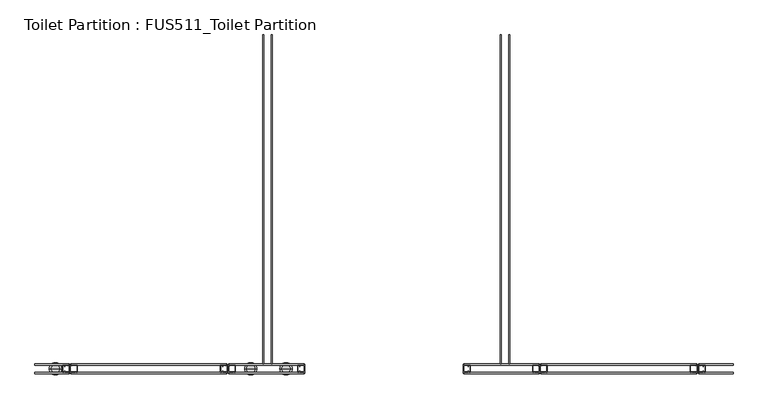
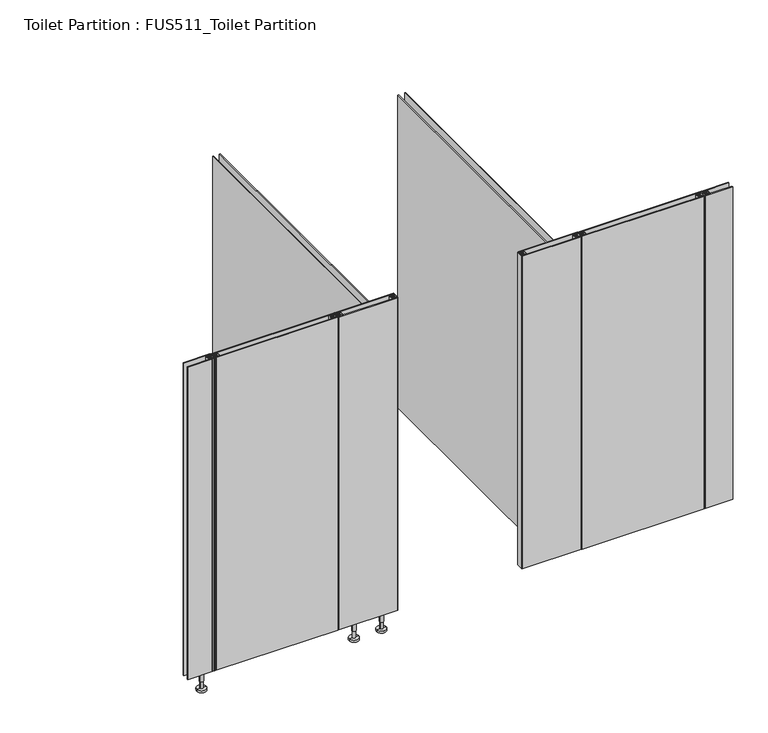
"""IFC4 building model written with IfcOpenShell, lengths in millimetres: furniture geometry, Toilet Partition : FUS511_Toilet Partition."""

from ifc_helpers import new_model, si_unit, point, frame, frame_2d, origin, place, context, project, spatial, polyline, circle_curve, trimmed, segment, composite_curve, outline, extrude, source, transform, mapped, element, save
from ifc_brep_helpers import plane_surface, cylinder_surface, advanced_brep


def toilet_partition_fus511_toilet_partition_2ff23377(model_context):
    return source(origin(), model_context, "Body", "SolidModel", [
        advanced_brep(
        [(-443.912605, 474.714347, 104.1461397), (-412.6687631, 474.714347, 104.1461397), (-412.6687631, 474.714347, 101.0217555), (-443.912605, 474.714347, 101.0217555), (-454.3272189, 474.714347, 0.0), (-402.2541491, 474.714347, 0.0), (-428.290684, 474.714347, 0.0), (-454.3272189, 474.714347, 10.414614), (-402.2541491, 474.714347, 10.414614), (-436.1016445, 474.714347, 10.414614), (-420.4797235, 474.714347, 10.414614), (-436.1016445, 474.714347, 52.0730698), (-420.4797235, 474.714347, 52.0730698), (-438.705298, 474.714347, 52.0730698), (-417.8760701, 474.714347, 52.0730698), (-438.705298, 474.714347, 101.0217555), (-417.8760701, 474.714347, 101.0217555), (-445.9955278, 474.714347, 104.1461397), (-410.5858403, 474.714347, 104.1461397), (-445.9955278, 474.714347, 110.394908), (-410.5858403, 474.714347, 110.394908), (-428.290684, 474.714347, 110.394908)],
        [
            (0, 1, circle_curve(frame((-428.290684, 474.714347, 104.1461397), z_axis=(0.0, 0.0, -1.0), x_axis=(1.0, 0.0, 0.0)), 15.6219209)),
            (1, 2),
            (2, 3, circle_curve(frame((-428.290684, 474.714347, 101.0217555), z_axis=(0.0, 0.0, 1.0), x_axis=(1.0, 0.0, 0.0)), 15.6219209)),
            (3, 0),
            (1, 0, circle_curve(frame((-428.290684, 474.714347, 104.1461397), z_axis=(0.0, 0.0, -1.0), x_axis=(1.0, 0.0, 0.0)), 15.6219209)),
            (3, 2, circle_curve(frame((-428.290684, 474.714347, 101.0217555), z_axis=(0.0, 0.0, 1.0), x_axis=(1.0, 0.0, 0.0)), 15.6219209)),
            (4, 5, circle_curve(frame((-428.290684, 474.714347, 0.0), z_axis=(0.0, 0.0, -1.0), x_axis=(1.0, 0.0, 0.0)), 26.0365349)),
            (5, 6),
            (6, 4),
            (5, 4, circle_curve(frame((-428.290684, 474.714347, 0.0), z_axis=(0.0, 0.0, -1.0), x_axis=(1.0, 0.0, 0.0)), 26.0365349)),
            (7, 8, circle_curve(frame((-428.290684, 474.714347, 10.414614), z_axis=(0.0, 0.0, -1.0), x_axis=(1.0, 0.0, 0.0)), 26.0365349)),
            (8, 5),
            (4, 7),
            (8, 7, circle_curve(frame((-428.290684, 474.714347, 10.414614), z_axis=(0.0, 0.0, -1.0), x_axis=(1.0, 0.0, 0.0)), 26.0365349)),
            (9, 10, circle_curve(frame((-428.290684, 474.714347, 10.414614), z_axis=(0.0, 0.0, -1.0), x_axis=(1.0, 0.0, 0.0)), 7.8109605)),
            (10, 8),
            (7, 9),
            (10, 9, circle_curve(frame((-428.290684, 474.714347, 10.414614), z_axis=(0.0, 0.0, -1.0), x_axis=(1.0, 0.0, 0.0)), 7.8109605)),
            (11, 12, circle_curve(frame((-428.290684, 474.714347, 52.0730698), z_axis=(0.0, 0.0, -1.0), x_axis=(1.0, 0.0, 0.0)), 7.8109605)),
            (12, 10),
            (9, 11),
            (12, 11, circle_curve(frame((-428.290684, 474.714347, 52.0730698), z_axis=(0.0, 0.0, -1.0), x_axis=(1.0, 0.0, 0.0)), 7.8109605)),
            (13, 14, circle_curve(frame((-428.290684, 474.714347, 52.0730698), z_axis=(0.0, 0.0, -1.0), x_axis=(1.0, 0.0, 0.0)), 10.414614)),
            (14, 12),
            (11, 13),
            (14, 13, circle_curve(frame((-428.290684, 474.714347, 52.0730698), z_axis=(0.0, 0.0, -1.0), x_axis=(1.0, 0.0, 0.0)), 10.414614)),
            (15, 16, circle_curve(frame((-428.290684, 474.714347, 101.0217555), z_axis=(0.0, 0.0, -1.0), x_axis=(1.0, 0.0, 0.0)), 10.414614)),
            (16, 14),
            (13, 15),
            (16, 15, circle_curve(frame((-428.290684, 474.714347, 101.0217555), z_axis=(0.0, 0.0, -1.0), x_axis=(1.0, 0.0, 0.0)), 10.414614)),
            (2, 16),
            (15, 3),
            (17, 18, circle_curve(frame((-428.290684, 474.714347, 104.1461397), z_axis=(0.0, 0.0, -1.0), x_axis=(1.0, 0.0, 0.0)), 17.7048437)),
            (18, 1),
            (0, 17),
            (18, 17, circle_curve(frame((-428.290684, 474.714347, 104.1461397), z_axis=(0.0, 0.0, -1.0), x_axis=(1.0, 0.0, 0.0)), 17.7048437)),
            (19, 20, circle_curve(frame((-428.290684, 474.714347, 110.394908), z_axis=(0.0, 0.0, -1.0), x_axis=(1.0, 0.0, 0.0)), 17.7048437)),
            (20, 18),
            (17, 19),
            (20, 19, circle_curve(frame((-428.290684, 474.714347, 110.394908), z_axis=(0.0, 0.0, -1.0), x_axis=(1.0, 0.0, 0.0)), 17.7048437)),
            (21, 20),
            (19, 21),
        ],
        [
            cylinder_surface(frame((-428.290684, 474.714347, 190.0), z_axis=(0.0, 0.0, 1.0), x_axis=(1.0, 0.0, 0.0)), 15.6219209),
            plane_surface(frame((-428.290684, 474.714347, 0.0), z_axis=(0.0, 0.0, -1.0), x_axis=(1.0, 0.0, 0.0))),
            cylinder_surface(frame((-428.290684, 474.714347, 190.0), z_axis=(0.0, 0.0, 1.0), x_axis=(1.0, 0.0, 0.0)), 26.0365349),
            plane_surface(frame((-428.290684, 474.714347, 10.414614), z_axis=(0.0, 0.0, 1.0), x_axis=(1.0, 0.0, 0.0))),
            cylinder_surface(frame((-428.290684, 474.714347, 190.0), z_axis=(0.0, 0.0, 1.0), x_axis=(1.0, 0.0, 0.0)), 7.8109605),
            plane_surface(frame((-428.290684, 474.714347, 52.0730698), z_axis=(0.0, 0.0, -1.0), x_axis=(1.0, 0.0, 0.0))),
            cylinder_surface(frame((-428.290684, 474.714347, 190.0), z_axis=(0.0, 0.0, 1.0), x_axis=(1.0, 0.0, 0.0)), 10.414614),
            plane_surface(frame((-428.290684, 474.714347, 101.0217555), z_axis=(0.0, 0.0, -1.0), x_axis=(1.0, 0.0, 0.0))),
            plane_surface(frame((-428.290684, 474.714347, 104.1461397), z_axis=(0.0, 0.0, -1.0), x_axis=(1.0, 0.0, 0.0))),
            cylinder_surface(frame((-428.290684, 474.714347, 190.0), z_axis=(0.0, 0.0, 1.0), x_axis=(1.0, 0.0, 0.0)), 17.7048437),
            plane_surface(frame((-428.290684, 474.714347, 110.394908), z_axis=(0.0, 0.0, 1.0), x_axis=(1.0, 0.0, 0.0))),
        ],
        [
            (0, [[1, 2, 3, 4]]),
            (0, [[5, -4, 6, -2]]),
            (1, [[7, 8, 9]]),
            (1, [[10, -9, -8]]),
            (2, [[11, 12, -7, 13]]),
            (2, [[14, -13, -10, -12]]),
            (3, [[15, 16, -11, 17]]),
            (3, [[18, -17, -14, -16]]),
            (4, [[19, 20, -15, 21]]),
            (4, [[22, -21, -18, -20]]),
            (5, [[23, 24, -19, 25]]),
            (5, [[26, -25, -22, -24]]),
            (6, [[27, 28, -23, 29]]),
            (6, [[30, -29, -26, -28]]),
            (7, [[-3, 31, -27, 32]]),
            (7, [[-6, -32, -30, -31]]),
            (8, [[33, 34, -1, 35]]),
            (8, [[36, -35, -5, -34]]),
            (9, [[37, 38, -33, 39]]),
            (9, [[40, -39, -36, -38]]),
            (10, [[41, -37, 42]]),
            (10, [[-42, -40, -41]]),
        ],
    ),
        advanced_brep(
        [(-593.912605, 474.714347, 104.1461397), (-562.6687631, 474.714347, 104.1461397), (-562.6687631, 474.714347, 101.0217555), (-593.912605, 474.714347, 101.0217555), (-604.3272189, 474.714347, 0.0), (-552.2541491, 474.714347, 0.0), (-578.290684, 474.714347, 0.0), (-604.3272189, 474.714347, 10.414614), (-552.2541491, 474.714347, 10.414614), (-586.1016445, 474.714347, 10.414614), (-570.4797235, 474.714347, 10.414614), (-586.1016445, 474.714347, 52.0730698), (-570.4797235, 474.714347, 52.0730698), (-588.705298, 474.714347, 52.0730698), (-567.8760701, 474.714347, 52.0730698), (-588.705298, 474.714347, 101.0217555), (-567.8760701, 474.714347, 101.0217555), (-595.9955278, 474.714347, 104.1461397), (-560.5858403, 474.714347, 104.1461397), (-595.9955278, 474.714347, 110.394908), (-560.5858403, 474.714347, 110.394908), (-578.290684, 474.714347, 110.394908)],
        [
            (0, 1, circle_curve(frame((-578.290684, 474.714347, 104.1461397), z_axis=(0.0, 0.0, -1.0), x_axis=(1.0, 0.0, 0.0)), 15.6219209)),
            (1, 2),
            (2, 3, circle_curve(frame((-578.290684, 474.714347, 101.0217555), z_axis=(0.0, 0.0, 1.0), x_axis=(1.0, 0.0, 0.0)), 15.6219209)),
            (3, 0),
            (1, 0, circle_curve(frame((-578.290684, 474.714347, 104.1461397), z_axis=(0.0, 0.0, -1.0), x_axis=(1.0, 0.0, 0.0)), 15.6219209)),
            (3, 2, circle_curve(frame((-578.290684, 474.714347, 101.0217555), z_axis=(0.0, 0.0, 1.0), x_axis=(1.0, 0.0, 0.0)), 15.6219209)),
            (4, 5, circle_curve(frame((-578.290684, 474.714347, 0.0), z_axis=(0.0, 0.0, -1.0), x_axis=(1.0, 0.0, 0.0)), 26.0365349)),
            (5, 6),
            (6, 4),
            (5, 4, circle_curve(frame((-578.290684, 474.714347, 0.0), z_axis=(0.0, 0.0, -1.0), x_axis=(1.0, 0.0, 0.0)), 26.0365349)),
            (7, 8, circle_curve(frame((-578.290684, 474.714347, 10.414614), z_axis=(0.0, 0.0, -1.0), x_axis=(1.0, 0.0, 0.0)), 26.0365349)),
            (8, 5),
            (4, 7),
            (8, 7, circle_curve(frame((-578.290684, 474.714347, 10.414614), z_axis=(0.0, 0.0, -1.0), x_axis=(1.0, 0.0, 0.0)), 26.0365349)),
            (9, 10, circle_curve(frame((-578.290684, 474.714347, 10.414614), z_axis=(0.0, 0.0, -1.0), x_axis=(1.0, 0.0, 0.0)), 7.8109605)),
            (10, 8),
            (7, 9),
            (10, 9, circle_curve(frame((-578.290684, 474.714347, 10.414614), z_axis=(0.0, 0.0, -1.0), x_axis=(1.0, 0.0, 0.0)), 7.8109605)),
            (11, 12, circle_curve(frame((-578.290684, 474.714347, 52.0730698), z_axis=(0.0, 0.0, -1.0), x_axis=(1.0, 0.0, 0.0)), 7.8109605)),
            (12, 10),
            (9, 11),
            (12, 11, circle_curve(frame((-578.290684, 474.714347, 52.0730698), z_axis=(0.0, 0.0, -1.0), x_axis=(1.0, 0.0, 0.0)), 7.8109605)),
            (13, 14, circle_curve(frame((-578.290684, 474.714347, 52.0730698), z_axis=(0.0, 0.0, -1.0), x_axis=(1.0, 0.0, 0.0)), 10.414614)),
            (14, 12),
            (11, 13),
            (14, 13, circle_curve(frame((-578.290684, 474.714347, 52.0730698), z_axis=(0.0, 0.0, -1.0), x_axis=(1.0, 0.0, 0.0)), 10.414614)),
            (15, 16, circle_curve(frame((-578.290684, 474.714347, 101.0217555), z_axis=(0.0, 0.0, -1.0), x_axis=(1.0, 0.0, 0.0)), 10.414614)),
            (16, 14),
            (13, 15),
            (16, 15, circle_curve(frame((-578.290684, 474.714347, 101.0217555), z_axis=(0.0, 0.0, -1.0), x_axis=(1.0, 0.0, 0.0)), 10.414614)),
            (2, 16),
            (15, 3),
            (17, 18, circle_curve(frame((-578.290684, 474.714347, 104.1461397), z_axis=(0.0, 0.0, -1.0), x_axis=(1.0, 0.0, 0.0)), 17.7048437)),
            (18, 1),
            (0, 17),
            (18, 17, circle_curve(frame((-578.290684, 474.714347, 104.1461397), z_axis=(0.0, 0.0, -1.0), x_axis=(1.0, 0.0, 0.0)), 17.7048437)),
            (19, 20, circle_curve(frame((-578.290684, 474.714347, 110.394908), z_axis=(0.0, 0.0, -1.0), x_axis=(1.0, 0.0, 0.0)), 17.7048437)),
            (20, 18),
            (17, 19),
            (20, 19, circle_curve(frame((-578.290684, 474.714347, 110.394908), z_axis=(0.0, 0.0, -1.0), x_axis=(1.0, 0.0, 0.0)), 17.7048437)),
            (21, 20),
            (19, 21),
        ],
        [
            cylinder_surface(frame((-578.290684, 474.714347, 190.0), z_axis=(0.0, 0.0, 1.0), x_axis=(1.0, 0.0, 0.0)), 15.6219209),
            plane_surface(frame((-578.290684, 474.714347, 0.0), z_axis=(0.0, 0.0, -1.0), x_axis=(1.0, 0.0, 0.0))),
            cylinder_surface(frame((-578.290684, 474.714347, 190.0), z_axis=(0.0, 0.0, 1.0), x_axis=(1.0, 0.0, 0.0)), 26.0365349),
            plane_surface(frame((-578.290684, 474.714347, 10.414614), z_axis=(0.0, 0.0, 1.0), x_axis=(1.0, 0.0, 0.0))),
            cylinder_surface(frame((-578.290684, 474.714347, 190.0), z_axis=(0.0, 0.0, 1.0), x_axis=(1.0, 0.0, 0.0)), 7.8109605),
            plane_surface(frame((-578.290684, 474.714347, 52.0730698), z_axis=(0.0, 0.0, -1.0), x_axis=(1.0, 0.0, 0.0))),
            cylinder_surface(frame((-578.290684, 474.714347, 190.0), z_axis=(0.0, 0.0, 1.0), x_axis=(1.0, 0.0, 0.0)), 10.414614),
            plane_surface(frame((-578.290684, 474.714347, 101.0217555), z_axis=(0.0, 0.0, -1.0), x_axis=(1.0, 0.0, 0.0))),
            plane_surface(frame((-578.290684, 474.714347, 104.1461397), z_axis=(0.0, 0.0, -1.0), x_axis=(1.0, 0.0, 0.0))),
            cylinder_surface(frame((-578.290684, 474.714347, 190.0), z_axis=(0.0, 0.0, 1.0), x_axis=(1.0, 0.0, 0.0)), 17.7048437),
            plane_surface(frame((-578.290684, 474.714347, 110.394908), z_axis=(0.0, 0.0, 1.0), x_axis=(1.0, 0.0, 0.0))),
        ],
        [
            (0, [[1, 2, 3, 4]]),
            (0, [[5, -4, 6, -2]]),
            (1, [[7, 8, 9]]),
            (1, [[10, -9, -8]]),
            (2, [[11, 12, -7, 13]]),
            (2, [[14, -13, -10, -12]]),
            (3, [[15, 16, -11, 17]]),
            (3, [[18, -17, -14, -16]]),
            (4, [[19, 20, -15, 21]]),
            (4, [[22, -21, -18, -20]]),
            (5, [[23, 24, -19, 25]]),
            (5, [[26, -25, -22, -24]]),
            (6, [[27, 28, -23, 29]]),
            (6, [[30, -29, -26, -28]]),
            (7, [[-3, 31, -27, 32]]),
            (7, [[-6, -32, -30, -31]]),
            (8, [[33, 34, -1, 35]]),
            (8, [[36, -35, -5, -34]]),
            (9, [[37, 38, -33, 39]]),
            (9, [[40, -39, -36, -38]]),
            (10, [[41, -37, 42]]),
            (10, [[-42, -40, -41]]),
        ],
    ),
        advanced_brep(
        [(-1423.912605, 474.714347, 104.1461397), (-1392.6687631, 474.714347, 104.1461397), (-1392.6687631, 474.714347, 101.0217555), (-1423.912605, 474.714347, 101.0217555), (-1434.3272189, 474.714347, 0.0), (-1382.2541491, 474.714347, 0.0), (-1408.290684, 474.714347, 0.0), (-1434.3272189, 474.714347, 10.414614), (-1382.2541491, 474.714347, 10.414614), (-1416.1016445, 474.714347, 10.414614), (-1400.4797235, 474.714347, 10.414614), (-1416.1016445, 474.714347, 52.0730698), (-1400.4797235, 474.714347, 52.0730698), (-1418.705298, 474.714347, 52.0730698), (-1397.8760701, 474.714347, 52.0730698), (-1418.705298, 474.714347, 101.0217555), (-1397.8760701, 474.714347, 101.0217555), (-1425.9955278, 474.714347, 104.1461397), (-1390.5858403, 474.714347, 104.1461397), (-1425.9955278, 474.714347, 110.394908), (-1390.5858403, 474.714347, 110.394908), (-1408.290684, 474.714347, 110.394908)],
        [
            (0, 1, circle_curve(frame((-1408.290684, 474.714347, 104.1461397), z_axis=(0.0, 0.0, -1.0), x_axis=(1.0, 0.0, 0.0)), 15.6219209)),
            (1, 2),
            (2, 3, circle_curve(frame((-1408.290684, 474.714347, 101.0217555), z_axis=(0.0, 0.0, 1.0), x_axis=(1.0, 0.0, 0.0)), 15.6219209)),
            (3, 0),
            (1, 0, circle_curve(frame((-1408.290684, 474.714347, 104.1461397), z_axis=(0.0, 0.0, -1.0), x_axis=(1.0, 0.0, 0.0)), 15.6219209)),
            (3, 2, circle_curve(frame((-1408.290684, 474.714347, 101.0217555), z_axis=(0.0, 0.0, 1.0), x_axis=(1.0, 0.0, 0.0)), 15.6219209)),
            (4, 5, circle_curve(frame((-1408.290684, 474.714347, 0.0), z_axis=(0.0, 0.0, -1.0), x_axis=(1.0, 0.0, 0.0)), 26.0365349)),
            (5, 6),
            (6, 4),
            (5, 4, circle_curve(frame((-1408.290684, 474.714347, 0.0), z_axis=(0.0, 0.0, -1.0), x_axis=(1.0, 0.0, 0.0)), 26.0365349)),
            (7, 8, circle_curve(frame((-1408.290684, 474.714347, 10.414614), z_axis=(0.0, 0.0, -1.0), x_axis=(1.0, 0.0, 0.0)), 26.0365349)),
            (8, 5),
            (4, 7),
            (8, 7, circle_curve(frame((-1408.290684, 474.714347, 10.414614), z_axis=(0.0, 0.0, -1.0), x_axis=(1.0, 0.0, 0.0)), 26.0365349)),
            (9, 10, circle_curve(frame((-1408.290684, 474.714347, 10.414614), z_axis=(0.0, 0.0, -1.0), x_axis=(1.0, 0.0, 0.0)), 7.8109605)),
            (10, 8),
            (7, 9),
            (10, 9, circle_curve(frame((-1408.290684, 474.714347, 10.414614), z_axis=(0.0, 0.0, -1.0), x_axis=(1.0, 0.0, 0.0)), 7.8109605)),
            (11, 12, circle_curve(frame((-1408.290684, 474.714347, 52.0730698), z_axis=(0.0, 0.0, -1.0), x_axis=(1.0, 0.0, 0.0)), 7.8109605)),
            (12, 10),
            (9, 11),
            (12, 11, circle_curve(frame((-1408.290684, 474.714347, 52.0730698), z_axis=(0.0, 0.0, -1.0), x_axis=(1.0, 0.0, 0.0)), 7.8109605)),
            (13, 14, circle_curve(frame((-1408.290684, 474.714347, 52.0730698), z_axis=(0.0, 0.0, -1.0), x_axis=(1.0, 0.0, 0.0)), 10.414614)),
            (14, 12),
            (11, 13),
            (14, 13, circle_curve(frame((-1408.290684, 474.714347, 52.0730698), z_axis=(0.0, 0.0, -1.0), x_axis=(1.0, 0.0, 0.0)), 10.414614)),
            (15, 16, circle_curve(frame((-1408.290684, 474.714347, 101.0217555), z_axis=(0.0, 0.0, -1.0), x_axis=(1.0, 0.0, 0.0)), 10.414614)),
            (16, 14),
            (13, 15),
            (16, 15, circle_curve(frame((-1408.290684, 474.714347, 101.0217555), z_axis=(0.0, 0.0, -1.0), x_axis=(1.0, 0.0, 0.0)), 10.414614)),
            (2, 16),
            (15, 3),
            (17, 18, circle_curve(frame((-1408.290684, 474.714347, 104.1461397), z_axis=(0.0, 0.0, -1.0), x_axis=(1.0, 0.0, 0.0)), 17.7048437)),
            (18, 1),
            (0, 17),
            (18, 17, circle_curve(frame((-1408.290684, 474.714347, 104.1461397), z_axis=(0.0, 0.0, -1.0), x_axis=(1.0, 0.0, 0.0)), 17.7048437)),
            (19, 20, circle_curve(frame((-1408.290684, 474.714347, 110.394908), z_axis=(0.0, 0.0, -1.0), x_axis=(1.0, 0.0, 0.0)), 17.7048437)),
            (20, 18),
            (17, 19),
            (20, 19, circle_curve(frame((-1408.290684, 474.714347, 110.394908), z_axis=(0.0, 0.0, -1.0), x_axis=(1.0, 0.0, 0.0)), 17.7048437)),
            (21, 20),
            (19, 21),
        ],
        [
            cylinder_surface(frame((-1408.290684, 474.714347, 190.0), z_axis=(0.0, 0.0, 1.0), x_axis=(1.0, 0.0, 0.0)), 15.6219209),
            plane_surface(frame((-1408.290684, 474.714347, 0.0), z_axis=(0.0, 0.0, -1.0), x_axis=(1.0, 0.0, 0.0))),
            cylinder_surface(frame((-1408.290684, 474.714347, 190.0), z_axis=(0.0, 0.0, 1.0), x_axis=(1.0, 0.0, 0.0)), 26.0365349),
            plane_surface(frame((-1408.290684, 474.714347, 10.414614), z_axis=(0.0, 0.0, 1.0), x_axis=(1.0, 0.0, 0.0))),
            cylinder_surface(frame((-1408.290684, 474.714347, 190.0), z_axis=(0.0, 0.0, 1.0), x_axis=(1.0, 0.0, 0.0)), 7.8109605),
            plane_surface(frame((-1408.290684, 474.714347, 52.0730698), z_axis=(0.0, 0.0, -1.0), x_axis=(1.0, 0.0, 0.0))),
            cylinder_surface(frame((-1408.290684, 474.714347, 190.0), z_axis=(0.0, 0.0, 1.0), x_axis=(1.0, 0.0, 0.0)), 10.414614),
            plane_surface(frame((-1408.290684, 474.714347, 101.0217555), z_axis=(0.0, 0.0, -1.0), x_axis=(1.0, 0.0, 0.0))),
            plane_surface(frame((-1408.290684, 474.714347, 104.1461397), z_axis=(0.0, 0.0, -1.0), x_axis=(1.0, 0.0, 0.0))),
            cylinder_surface(frame((-1408.290684, 474.714347, 190.0), z_axis=(0.0, 0.0, 1.0), x_axis=(1.0, 0.0, 0.0)), 17.7048437),
            plane_surface(frame((-1408.290684, 474.714347, 110.394908), z_axis=(0.0, 0.0, 1.0), x_axis=(1.0, 0.0, 0.0))),
        ],
        [
            (0, [[1, 2, 3, 4]]),
            (0, [[5, -4, 6, -2]]),
            (1, [[7, 8, 9]]),
            (1, [[10, -9, -8]]),
            (2, [[11, 12, -7, 13]]),
            (2, [[14, -13, -10, -12]]),
            (3, [[15, 16, -11, 17]]),
            (3, [[18, -17, -14, -16]]),
            (4, [[19, 20, -15, 21]]),
            (4, [[22, -21, -18, -20]]),
            (5, [[23, 24, -19, 25]]),
            (5, [[26, -25, -22, -24]]),
            (6, [[27, 28, -23, 29]]),
            (6, [[30, -29, -26, -28]]),
            (7, [[-3, 31, -27, 32]]),
            (7, [[-6, -32, -30, -31]]),
            (8, [[33, 34, -1, 35]]),
            (8, [[36, -35, -5, -34]]),
            (9, [[37, 38, -33, 39]]),
            (9, [[40, -39, -36, -38]]),
            (10, [[41, -37, 42]]),
            (10, [[-42, -40, -41]]),
        ],
    ),
        extrude(outline(polyline([(-486.6876721, 495.214347), (-491.6876721, 495.214347), (-491.6876721, 1895.214347), (-486.6876721, 1895.214347), (-486.6876721, 495.214347)])), frame((0.0, 0.0, 100.0), z_axis=(0.0, 0.0, 1.0), x_axis=(1.0, 0.0, 0.0)), (0.0, 0.0, 1.0), 1800.0),
        extrude(outline(polyline([(-522.6876721, 495.214347), (-527.6876721, 495.214347), (-527.6876721, 1895.214347), (-522.6876721, 1895.214347), (-522.6876721, 495.214347)])), frame((0.0, 0.0, 100.0), z_axis=(0.0, 0.0, 1.0), x_axis=(1.0, 0.0, 0.0)), (0.0, 0.0, 1.0), 1800.0),
        extrude(outline(polyline([(522.879415, 495.214347), (517.879415, 495.214347), (517.879415, 1895.214347), (522.879415, 1895.214347), (522.879415, 495.214347)])), frame((0.0, 0.0, 100.0), z_axis=(0.0, 0.0, 1.0), x_axis=(1.0, 0.0, 0.0)), (0.0, 0.0, 1.0), 1800.0),
        extrude(outline(polyline([(486.879415, 495.214347), (481.879415, 495.214347), (481.879415, 1895.214347), (486.879415, 1895.214347), (486.879415, 495.214347)])), frame((0.0, 0.0, 100.0), z_axis=(0.0, 0.0, 1.0), x_axis=(1.0, 0.0, 0.0)), (0.0, 0.0, 1.0), 1800.0),
        extrude(outline(composite_curve([segment(polyline([(1354.2282685, 489.5206414), (1354.2282685, 459.9080525), (1349.292837, 459.9080525), (1349.292837, 460.8951388), (1345.3444919, 460.8951388), (1345.3444919, 459.9080525), (1331.7720553, 459.9080525)]), True, "CONTINUOUS"), segment(trimmed(circle_curve(frame_2d((1331.5252837, 460.8637947)), 0.9870863), [point((1331.7720553, 459.9080525))], [point((1331.2785121, 459.9080525))], True, "CARTESIAN"), True, "CONTINUOUS"), segment(polyline([(1331.2785121, 459.9080525), (1326.5898522, 459.9080525), (1326.5898522, 454.9726211), (1325.6027659, 454.9726211)]), True, "CONTINUOUS"), segment(trimmed(circle_curve(frame_2d((1325.6027659, 455.9597074)), 0.9870863), [point((1325.6027659, 454.9726211))], [point((1324.6156797, 455.9597074))], False, "CARTESIAN"), True, "CONTINUOUS"), segment(polyline([(1324.6156797, 455.9597074), (1324.6156797, 493.4689866)]), True, "CONTINUOUS"), segment(trimmed(circle_curve(frame_2d((1325.6027659, 493.4689866)), 0.9870863), [point((1324.6156797, 493.4689866))], [point((1325.6027659, 494.4560729))], False, "CARTESIAN"), True, "CONTINUOUS"), segment(polyline([(1325.6027659, 494.4560729), (1326.5898522, 494.4560729), (1326.5898522, 489.5206414), (1331.2785121, 489.5206414)]), True, "CONTINUOUS"), segment(trimmed(circle_curve(frame_2d((1331.5252837, 488.5648992)), 0.9870863), [point((1331.2785121, 489.5206414))], [point((1331.7720553, 489.5206414))], True, "CARTESIAN"), True, "CONTINUOUS"), segment(polyline([(1331.7720553, 489.5206414), (1345.3444919, 488.5335551), (1349.292837, 488.5335551), (1349.292837, 489.5206414), (1354.2282685, 489.5206414)]), True, "CONTINUOUS")], self_intersect=False), holes=[polyline([(1351.2670096, 486.5593825), (1346.3315781, 486.5593825), (1346.3315781, 481.623951), (1343.3703193, 481.623951), (1343.3703193, 486.5593825), (1336.4607152, 486.5593825), (1336.4607152, 482.1174942), (1334.9800858, 482.1174942), (1334.9800858, 486.5593825), (1333.2526847, 486.5593825), (1333.2526847, 484.5852099), (1329.3043396, 484.5852099), (1329.3043396, 486.5593825), (1327.5769385, 486.5593825), (1327.5769385, 462.8693114), (1329.3043396, 462.8693114), (1329.3043396, 464.843484), (1333.2526847, 464.843484), (1333.2526847, 462.8693114), (1334.9800858, 462.8693114), (1334.9800858, 467.3111998), (1336.4607152, 467.3111998), (1336.4607152, 462.8693114), (1343.3703193, 462.8693114), (1343.3703193, 467.8047429), (1346.3315781, 467.8047429), (1346.3315781, 462.8693114), (1351.2670096, 462.8693114), (1351.2670096, 486.5593825)])]), frame((0.0, 0.0, 100.0), z_axis=(0.0, 0.0, 1.0), x_axis=(1.0, 0.0, 0.0)), (0.0, 0.0, 1.0), 1800.0),
        extrude(outline(polyline([(1471.5898522, 454.214347), (1326.5898522, 454.214347), (1326.5898522, 459.214347), (1471.5898522, 459.214347), (1471.5898522, 454.214347)])), frame((0.0, 0.0, 100.0), z_axis=(0.0, 0.0, 1.0), x_axis=(1.0, 0.0, 0.0)), (0.0, 0.0, 1.0), 1800.0),
        extrude(outline(polyline([(1471.5898522, 490.214347), (1326.5898522, 490.214347), (1326.5898522, 495.214347), (1471.5898522, 495.214347), (1471.5898522, 490.214347)])), frame((0.0, 0.0, 100.0), z_axis=(0.0, 0.0, 1.0), x_axis=(1.0, 0.0, 0.0)), (0.0, 0.0, 1.0), 1800.0),
        extrude(outline(composite_curve([segment(polyline([(681.0354151, 489.5206414), (681.0354151, 459.9080525), (676.0999837, 459.9080525), (676.0999837, 460.8951388), (672.1516385, 460.8951388), (672.1516385, 459.9080525), (658.5792019, 459.9080525)]), True, "CONTINUOUS"), segment(trimmed(circle_curve(frame_2d((658.3324304, 460.8637947)), 0.9870863), [point((658.5792019, 459.9080525))], [point((658.0856588, 459.9080525))], True, "CARTESIAN"), True, "CONTINUOUS"), segment(polyline([(658.0856588, 459.9080525), (653.3969989, 459.9080525), (653.3969989, 454.9726211), (652.4099126, 454.9726211)]), True, "CONTINUOUS"), segment(trimmed(circle_curve(frame_2d((652.4099126, 455.9597074)), 0.9870863), [point((652.4099126, 454.9726211))], [point((651.4228263, 455.9597074))], False, "CARTESIAN"), True, "CONTINUOUS"), segment(polyline([(651.4228263, 455.9597074), (651.4228263, 493.4689866)]), True, "CONTINUOUS"), segment(trimmed(circle_curve(frame_2d((652.4099126, 493.4689866)), 0.9870863), [point((651.4228263, 493.4689866))], [point((652.4099126, 494.4560729))], False, "CARTESIAN"), True, "CONTINUOUS"), segment(polyline([(652.4099126, 494.4560729), (653.3969989, 494.4560729), (653.3969989, 489.5206414), (658.0856588, 489.5206414)]), True, "CONTINUOUS"), segment(trimmed(circle_curve(frame_2d((658.3324304, 488.5648992)), 0.9870863), [point((658.0856588, 489.5206414))], [point((658.5792019, 489.5206414))], True, "CARTESIAN"), True, "CONTINUOUS"), segment(polyline([(658.5792019, 489.5206414), (672.1516385, 488.5335551), (676.0999837, 488.5335551), (676.0999837, 489.5206414), (681.0354151, 489.5206414)]), True, "CONTINUOUS")], self_intersect=False), holes=[polyline([(678.0741563, 486.5593825), (673.1387248, 486.5593825), (673.1387248, 481.623951), (670.1774659, 481.623951), (670.1774659, 486.5593825), (663.2678618, 486.5593825), (663.2678618, 482.1174942), (661.7872324, 482.1174942), (661.7872324, 486.5593825), (660.0598314, 486.5593825), (660.0598314, 484.5852099), (656.1114862, 484.5852099), (656.1114862, 486.5593825), (654.3840852, 486.5593825), (654.3840852, 462.8693114), (656.1114862, 462.8693114), (656.1114862, 464.843484), (660.0598314, 464.843484), (660.0598314, 462.8693114), (661.7872324, 462.8693114), (661.7872324, 467.3111998), (663.2678618, 467.3111998), (663.2678618, 462.8693114), (670.1774659, 462.8693114), (670.1774659, 467.8047429), (673.1387248, 467.8047429), (673.1387248, 462.8693114), (678.0741563, 462.8693114), (678.0741563, 486.5593825)])]), frame((0.0, 0.0, 100.0), z_axis=(0.0, 0.0, 1.0), x_axis=(1.0, 0.0, 0.0)), (0.0, 0.0, 1.0), 1800.0),
        extrude(outline(composite_curve([segment(polyline([(1289.7585826, 489.5206414), (1294.6940141, 489.5206414), (1294.6940141, 488.5335551), (1298.6423593, 488.5335551), (1312.2147958, 489.5206414)]), True, "CONTINUOUS"), segment(trimmed(circle_curve(frame_2d((1312.4615674, 488.5648992)), 0.9870863), [point((1312.2147958, 489.5206414))], [point((1312.708339, 489.5206414))], True, "CARTESIAN"), True, "CONTINUOUS"), segment(polyline([(1312.708339, 489.5206414), (1317.3969989, 489.5206414), (1317.3969989, 494.4560729), (1318.3840852, 494.4560729)]), True, "CONTINUOUS"), segment(trimmed(circle_curve(frame_2d((1318.3840852, 493.4689866)), 0.9870863), [point((1318.3840852, 494.4560729))], [point((1319.3711715, 493.4689866))], False, "CARTESIAN"), True, "CONTINUOUS"), segment(polyline([(1319.3711715, 493.4689866), (1319.3711715, 455.9597074)]), True, "CONTINUOUS"), segment(trimmed(circle_curve(frame_2d((1318.3840852, 455.9597074)), 0.9870863), [point((1319.3711715, 455.9597074))], [point((1318.3840852, 454.9726211))], False, "CARTESIAN"), True, "CONTINUOUS"), segment(polyline([(1318.3840852, 454.9726211), (1317.3969989, 454.9726211), (1317.3969989, 459.9080525), (1312.708339, 459.9080525)]), True, "CONTINUOUS"), segment(trimmed(circle_curve(frame_2d((1312.4615674, 460.8637947)), 0.9870863), [point((1312.708339, 459.9080525))], [point((1312.2147958, 459.9080525))], True, "CARTESIAN"), True, "CONTINUOUS"), segment(polyline([(1312.2147958, 459.9080525), (1298.6423593, 459.9080525), (1298.6423593, 460.8951388), (1294.6940141, 460.8951388), (1294.6940141, 459.9080525), (1289.7585826, 459.9080525), (1289.7585826, 489.5206414)]), True, "CONTINUOUS")], self_intersect=False), holes=[polyline([(1292.7198415, 486.5593825), (1292.7198415, 462.8693114), (1297.655273, 462.8693114), (1297.655273, 467.8047429), (1300.6165319, 467.8047429), (1300.6165319, 462.8693114), (1307.5261359, 462.8693114), (1307.5261359, 467.3111998), (1309.0067654, 467.3111998), (1309.0067654, 462.8693114), (1310.7341664, 462.8693114), (1310.7341664, 464.843484), (1314.6825116, 464.843484), (1314.6825116, 462.8693114), (1316.4099126, 462.8693114), (1316.4099126, 486.5593825), (1314.6825116, 486.5593825), (1314.6825116, 484.5852099), (1310.7341664, 484.5852099), (1310.7341664, 486.5593825), (1309.0067654, 486.5593825), (1309.0067654, 482.1174942), (1307.5261359, 482.1174942), (1307.5261359, 486.5593825), (1300.6165319, 486.5593825), (1300.6165319, 481.623951), (1297.655273, 481.623951), (1297.655273, 486.5593825), (1292.7198415, 486.5593825)])]), frame((0.0, 0.0, 100.0), z_axis=(0.0, 0.0, 1.0), x_axis=(1.0, 0.0, 0.0)), (0.0, 0.0, 1.0), 1800.0),
        extrude(outline(polyline([(653.3969989, 454.214347), (653.3969989, 459.214347), (1317.3969989, 459.214347), (1317.3969989, 454.214347), (653.3969989, 454.214347)])), frame((0.0, 0.0, 100.0), z_axis=(0.0, 0.0, 1.0), x_axis=(1.0, 0.0, 0.0)), (0.0, 0.0, 1.0), 1800.0),
        extrude(outline(polyline([(653.3969989, 490.214347), (653.3969989, 495.214347), (1317.3969989, 495.214347), (1317.3969989, 490.214347), (653.3969989, 490.214347)])), frame((0.0, 0.0, 100.0), z_axis=(0.0, 0.0, 1.0), x_axis=(1.0, 0.0, 0.0)), (0.0, 0.0, 1.0), 1800.0),
        extrude(outline(composite_curve([segment(polyline([(355.296938, 489.5206414), (355.296938, 459.9080525), (350.3615065, 459.9080525), (350.3615065, 460.8951388), (346.4131614, 460.8951388), (346.4131614, 459.9080525), (332.8407248, 459.9080525)]), True, "CONTINUOUS"), segment(trimmed(circle_curve(frame_2d((332.5939532, 460.8637947)), 0.9870863), [point((332.8407248, 459.9080525))], [point((332.3471816, 459.9080525))], True, "CARTESIAN"), True, "CONTINUOUS"), segment(polyline([(332.3471816, 459.9080525), (327.6585217, 459.9080525), (327.6585217, 454.9726211), (326.6714355, 454.9726211)]), True, "CONTINUOUS"), segment(trimmed(circle_curve(frame_2d((326.6714355, 455.9597074)), 0.9870863), [point((326.6714355, 454.9726211))], [point((325.6843492, 455.9597074))], False, "CARTESIAN"), True, "CONTINUOUS"), segment(polyline([(325.6843492, 455.9597074), (325.6843492, 493.4689866)]), True, "CONTINUOUS"), segment(trimmed(circle_curve(frame_2d((326.6714355, 493.4689866)), 0.9870863), [point((325.6843492, 493.4689866))], [point((326.6714355, 494.4560729))], False, "CARTESIAN"), True, "CONTINUOUS"), segment(polyline([(326.6714355, 494.4560729), (327.6585217, 494.4560729), (327.6585217, 489.5206414), (332.3471816, 489.5206414)]), True, "CONTINUOUS"), segment(trimmed(circle_curve(frame_2d((332.5939532, 488.5648992)), 0.9870863), [point((332.3471816, 489.5206414))], [point((332.8407248, 489.5206414))], True, "CARTESIAN"), True, "CONTINUOUS"), segment(polyline([(332.8407248, 489.5206414), (346.4131614, 488.5335551), (350.3615065, 488.5335551), (350.3615065, 489.5206414), (355.296938, 489.5206414)]), True, "CONTINUOUS")], self_intersect=False), holes=[polyline([(352.3356791, 486.5593825), (347.4002477, 486.5593825), (347.4002477, 481.623951), (344.4389888, 481.623951), (344.4389888, 486.5593825), (337.5293847, 486.5593825), (337.5293847, 482.1174942), (336.0487553, 482.1174942), (336.0487553, 486.5593825), (334.3213542, 486.5593825), (334.3213542, 484.5852099), (330.3730091, 484.5852099), (330.3730091, 486.5593825), (328.645608, 486.5593825), (328.645608, 462.8693114), (330.3730091, 462.8693114), (330.3730091, 464.843484), (334.3213542, 464.843484), (334.3213542, 462.8693114), (336.0487553, 462.8693114), (336.0487553, 467.3111998), (337.5293847, 467.3111998), (337.5293847, 462.8693114), (344.4389888, 462.8693114), (344.4389888, 467.8047429), (347.4002477, 467.8047429), (347.4002477, 462.8693114), (352.3356791, 462.8693114), (352.3356791, 486.5593825)])]), frame((0.0, 0.0, 100.0), z_axis=(0.0, 0.0, 1.0), x_axis=(1.0, 0.0, 0.0)), (0.0, 0.0, 1.0), 1800.0),
        extrude(outline(composite_curve([segment(polyline([(620.0201055, 489.5206414), (624.955537, 489.5206414), (624.955537, 488.5335551), (628.9038821, 488.5335551), (642.4763187, 489.5206414)]), True, "CONTINUOUS"), segment(trimmed(circle_curve(frame_2d((642.7230903, 488.5648992)), 0.9870863), [point((642.4763187, 489.5206414))], [point((642.9698618, 489.5206414))], True, "CARTESIAN"), True, "CONTINUOUS"), segment(polyline([(642.9698618, 489.5206414), (647.6585217, 489.5206414), (647.6585217, 494.4560729), (648.645608, 494.4560729)]), True, "CONTINUOUS"), segment(trimmed(circle_curve(frame_2d((648.645608, 493.4689866)), 0.9870863), [point((648.645608, 494.4560729))], [point((649.6326943, 493.4689866))], False, "CARTESIAN"), True, "CONTINUOUS"), segment(polyline([(649.6326943, 493.4689866), (649.6326943, 455.9597074)]), True, "CONTINUOUS"), segment(trimmed(circle_curve(frame_2d((648.645608, 455.9597074)), 0.9870863), [point((649.6326943, 455.9597074))], [point((648.645608, 454.9726211))], False, "CARTESIAN"), True, "CONTINUOUS"), segment(polyline([(648.645608, 454.9726211), (647.6585217, 454.9726211), (647.6585217, 459.9080525), (642.9698618, 459.9080525)]), True, "CONTINUOUS"), segment(trimmed(circle_curve(frame_2d((642.7230903, 460.8637947)), 0.9870863), [point((642.9698618, 459.9080525))], [point((642.4763187, 459.9080525))], True, "CARTESIAN"), True, "CONTINUOUS"), segment(polyline([(642.4763187, 459.9080525), (628.9038821, 459.9080525), (628.9038821, 460.8951388), (624.955537, 460.8951388), (624.955537, 459.9080525), (620.0201055, 459.9080525), (620.0201055, 489.5206414)]), True, "CONTINUOUS")], self_intersect=False), holes=[polyline([(622.9813644, 486.5593825), (622.9813644, 462.8693114), (627.9167958, 462.8693114), (627.9167958, 467.8047429), (630.8780547, 467.8047429), (630.8780547, 462.8693114), (637.7876588, 462.8693114), (637.7876588, 467.3111998), (639.2682882, 467.3111998), (639.2682882, 462.8693114), (640.9956893, 462.8693114), (640.9956893, 464.843484), (644.9440344, 464.843484), (644.9440344, 462.8693114), (646.6714355, 462.8693114), (646.6714355, 486.5593825), (644.9440344, 486.5593825), (644.9440344, 484.5852099), (640.9956893, 484.5852099), (640.9956893, 486.5593825), (639.2682882, 486.5593825), (639.2682882, 482.1174942), (637.7876588, 482.1174942), (637.7876588, 486.5593825), (630.8780547, 486.5593825), (630.8780547, 481.623951), (627.9167958, 481.623951), (627.9167958, 486.5593825), (622.9813644, 486.5593825)])]), frame((0.0, 0.0, 100.0), z_axis=(0.0, 0.0, 1.0), x_axis=(1.0, 0.0, 0.0)), (0.0, 0.0, 1.0), 1800.0),
        extrude(outline(polyline([(327.6585217, 454.214347), (327.6585217, 459.214347), (647.6585217, 459.214347), (647.6585217, 454.214347), (327.6585217, 454.214347)])), frame((0.0, 0.0, 100.0), z_axis=(0.0, 0.0, 1.0), x_axis=(1.0, 0.0, 0.0)), (0.0, 0.0, 1.0), 1800.0),
        extrude(outline(polyline([(327.6585217, 490.214347), (327.6585217, 495.214347), (647.6585217, 495.214347), (647.6585217, 490.214347), (327.6585217, 490.214347)])), frame((0.0, 0.0, 100.0), z_axis=(0.0, 0.0, 1.0), x_axis=(1.0, 0.0, 0.0)), (0.0, 0.0, 1.0), 1800.0),
        extrude(outline(composite_curve([segment(polyline([(-1378.0265961, 489.5206414), (-1373.0911646, 489.5206414), (-1373.0911646, 488.5335551), (-1369.1428194, 488.5335551), (-1355.5703828, 489.5206414)]), True, "CONTINUOUS"), segment(trimmed(circle_curve(frame_2d((-1355.3236113, 488.5648992)), 0.9870863), [point((-1355.5703828, 489.5206414))], [point((-1355.0768397, 489.5206414))], True, "CARTESIAN"), True, "CONTINUOUS"), segment(polyline([(-1355.0768397, 489.5206414), (-1350.3881798, 489.5206414), (-1350.3881798, 494.4560729), (-1349.4010935, 494.4560729)]), True, "CONTINUOUS"), segment(trimmed(circle_curve(frame_2d((-1349.4010935, 493.4689866)), 0.9870863), [point((-1349.4010935, 494.4560729))], [point((-1348.4140072, 493.4689866))], False, "CARTESIAN"), True, "CONTINUOUS"), segment(polyline([(-1348.4140072, 493.4689866), (-1348.4140072, 455.9597074)]), True, "CONTINUOUS"), segment(trimmed(circle_curve(frame_2d((-1349.4010935, 455.9597074)), 0.9870863), [point((-1348.4140072, 455.9597074))], [point((-1349.4010935, 454.9726211))], False, "CARTESIAN"), True, "CONTINUOUS"), segment(polyline([(-1349.4010935, 454.9726211), (-1350.3881798, 454.9726211), (-1350.3881798, 459.9080525), (-1355.0768397, 459.9080525)]), True, "CONTINUOUS"), segment(trimmed(circle_curve(frame_2d((-1355.3236113, 460.8637947)), 0.9870863), [point((-1355.0768397, 459.9080525))], [point((-1355.5703828, 459.9080525))], True, "CARTESIAN"), True, "CONTINUOUS"), segment(polyline([(-1355.5703828, 459.9080525), (-1369.1428194, 459.9080525), (-1369.1428194, 460.8951388), (-1373.0911646, 460.8951388), (-1373.0911646, 459.9080525), (-1378.0265961, 459.9080525), (-1378.0265961, 489.5206414)]), True, "CONTINUOUS")], self_intersect=False), holes=[polyline([(-1375.0653372, 486.5593825), (-1375.0653372, 462.8693114), (-1370.1299057, 462.8693114), (-1370.1299057, 467.8047429), (-1367.1686468, 467.8047429), (-1367.1686468, 462.8693114), (-1360.2590427, 462.8693114), (-1360.2590427, 467.3111998), (-1358.7784133, 467.3111998), (-1358.7784133, 462.8693114), (-1357.0510123, 462.8693114), (-1357.0510123, 464.843484), (-1353.1026671, 464.843484), (-1353.1026671, 462.8693114), (-1351.3752661, 462.8693114), (-1351.3752661, 486.5593825), (-1353.1026671, 486.5593825), (-1353.1026671, 484.5852099), (-1357.0510123, 484.5852099), (-1357.0510123, 486.5593825), (-1358.7784133, 486.5593825), (-1358.7784133, 482.1174942), (-1360.2590427, 482.1174942), (-1360.2590427, 486.5593825), (-1367.1686468, 486.5593825), (-1367.1686468, 481.623951), (-1370.1299057, 481.623951), (-1370.1299057, 486.5593825), (-1375.0653372, 486.5593825)])]), frame((0.0, 0.0, 100.0), z_axis=(0.0, 0.0, 1.0), x_axis=(1.0, 0.0, 0.0)), (0.0, 0.0, 1.0), 1800.0),
        extrude(outline(polyline([(-1495.3881798, 454.214347), (-1495.3881798, 459.214347), (-1350.3881798, 459.214347), (-1350.3881798, 454.214347), (-1495.3881798, 454.214347)])), frame((0.0, 0.0, 100.0), z_axis=(0.0, 0.0, 1.0), x_axis=(1.0, 0.0, 0.0)), (0.0, 0.0, 1.0), 1800.0),
        extrude(outline(polyline([(-1495.3881798, 490.214347), (-1495.3881798, 495.214347), (-1350.3881798, 495.214347), (-1350.3881798, 490.214347), (-1495.3881798, 490.214347)])), frame((0.0, 0.0, 100.0), z_axis=(0.0, 0.0, 1.0), x_axis=(1.0, 0.0, 0.0)), (0.0, 0.0, 1.0), 1800.0),
        extrude(outline(composite_curve([segment(polyline([(-1315.5310829, 489.5206414), (-1315.5310829, 459.9080525), (-1320.4665144, 459.9080525), (-1320.4665144, 460.8951388), (-1324.4148596, 460.8951388), (-1324.4148596, 459.9080525), (-1337.9872961, 459.9080525)]), True, "CONTINUOUS"), segment(trimmed(circle_curve(frame_2d((-1338.2340677, 460.8637947)), 0.9870863), [point((-1337.9872961, 459.9080525))], [point((-1338.4808393, 459.9080525))], True, "CARTESIAN"), True, "CONTINUOUS"), segment(polyline([(-1338.4808393, 459.9080525), (-1343.1694992, 459.9080525), (-1343.1694992, 454.9726211), (-1344.1565855, 454.9726211)]), True, "CONTINUOUS"), segment(trimmed(circle_curve(frame_2d((-1344.1565855, 455.9597074)), 0.9870863), [point((-1344.1565855, 454.9726211))], [point((-1345.1436718, 455.9597074))], False, "CARTESIAN"), True, "CONTINUOUS"), segment(polyline([(-1345.1436718, 455.9597074), (-1345.1436718, 493.4689866)]), True, "CONTINUOUS"), segment(trimmed(circle_curve(frame_2d((-1344.1565855, 493.4689866)), 0.9870863), [point((-1345.1436718, 493.4689866))], [point((-1344.1565855, 494.4560729))], False, "CARTESIAN"), True, "CONTINUOUS"), segment(polyline([(-1344.1565855, 494.4560729), (-1343.1694992, 494.4560729), (-1343.1694992, 489.5206414), (-1338.4808393, 489.5206414)]), True, "CONTINUOUS"), segment(trimmed(circle_curve(frame_2d((-1338.2340677, 488.5648992)), 0.9870863), [point((-1338.4808393, 489.5206414))], [point((-1337.9872961, 489.5206414))], True, "CARTESIAN"), True, "CONTINUOUS"), segment(polyline([(-1337.9872961, 489.5206414), (-1324.4148596, 488.5335551), (-1320.4665144, 488.5335551), (-1320.4665144, 489.5206414), (-1315.5310829, 489.5206414)]), True, "CONTINUOUS")], self_intersect=False), holes=[polyline([(-1318.4923418, 486.5593825), (-1323.4277733, 486.5593825), (-1323.4277733, 481.623951), (-1326.3890322, 481.623951), (-1326.3890322, 486.5593825), (-1333.2986362, 486.5593825), (-1333.2986362, 482.1174942), (-1334.7792657, 482.1174942), (-1334.7792657, 486.5593825), (-1336.5066667, 486.5593825), (-1336.5066667, 484.5852099), (-1340.4550119, 484.5852099), (-1340.4550119, 486.5593825), (-1342.1824129, 486.5593825), (-1342.1824129, 462.8693114), (-1340.4550119, 462.8693114), (-1340.4550119, 464.843484), (-1336.5066667, 464.843484), (-1336.5066667, 462.8693114), (-1334.7792657, 462.8693114), (-1334.7792657, 467.3111998), (-1333.2986362, 467.3111998), (-1333.2986362, 462.8693114), (-1326.3890322, 462.8693114), (-1326.3890322, 467.8047429), (-1323.4277733, 467.8047429), (-1323.4277733, 462.8693114), (-1318.4923418, 462.8693114), (-1318.4923418, 486.5593825)])]), frame((0.0, 0.0, 100.0), z_axis=(0.0, 0.0, 1.0), x_axis=(1.0, 0.0, 0.0)), (0.0, 0.0, 1.0), 1800.0),
        extrude(outline(composite_curve([segment(polyline([(-706.8079154, 489.5206414), (-701.872484, 489.5206414), (-701.872484, 488.5335551), (-697.9241388, 488.5335551), (-684.3517022, 489.5206414)]), True, "CONTINUOUS"), segment(trimmed(circle_curve(frame_2d((-684.1049306, 488.5648992)), 0.9870863), [point((-684.3517022, 489.5206414))], [point((-683.8581591, 489.5206414))], True, "CARTESIAN"), True, "CONTINUOUS"), segment(polyline([(-683.8581591, 489.5206414), (-679.1694992, 489.5206414), (-679.1694992, 494.4560729), (-678.1824129, 494.4560729)]), True, "CONTINUOUS"), segment(trimmed(circle_curve(frame_2d((-678.1824129, 493.4689866)), 0.9870863), [point((-678.1824129, 494.4560729))], [point((-677.1953266, 493.4689866))], False, "CARTESIAN"), True, "CONTINUOUS"), segment(polyline([(-677.1953266, 493.4689866), (-677.1953266, 455.9597074)]), True, "CONTINUOUS"), segment(trimmed(circle_curve(frame_2d((-678.1824129, 455.9597074)), 0.9870863), [point((-677.1953266, 455.9597074))], [point((-678.1824129, 454.9726211))], False, "CARTESIAN"), True, "CONTINUOUS"), segment(polyline([(-678.1824129, 454.9726211), (-679.1694992, 454.9726211), (-679.1694992, 459.9080525), (-683.8581591, 459.9080525)]), True, "CONTINUOUS"), segment(trimmed(circle_curve(frame_2d((-684.1049306, 460.8637947)), 0.9870863), [point((-683.8581591, 459.9080525))], [point((-684.3517022, 459.9080525))], True, "CARTESIAN"), True, "CONTINUOUS"), segment(polyline([(-684.3517022, 459.9080525), (-697.9241388, 459.9080525), (-697.9241388, 460.8951388), (-701.872484, 460.8951388), (-701.872484, 459.9080525), (-706.8079154, 459.9080525), (-706.8079154, 489.5206414)]), True, "CONTINUOUS")], self_intersect=False), holes=[polyline([(-703.8466566, 486.5593825), (-703.8466566, 462.8693114), (-698.9112251, 462.8693114), (-698.9112251, 467.8047429), (-695.9499662, 467.8047429), (-695.9499662, 462.8693114), (-689.0403621, 462.8693114), (-689.0403621, 467.3111998), (-687.5597327, 467.3111998), (-687.5597327, 462.8693114), (-685.8323317, 462.8693114), (-685.8323317, 464.843484), (-681.8839865, 464.843484), (-681.8839865, 462.8693114), (-680.1565855, 462.8693114), (-680.1565855, 486.5593825), (-681.8839865, 486.5593825), (-681.8839865, 484.5852099), (-685.8323317, 484.5852099), (-685.8323317, 486.5593825), (-687.5597327, 486.5593825), (-687.5597327, 482.1174942), (-689.0403621, 482.1174942), (-689.0403621, 486.5593825), (-695.9499662, 486.5593825), (-695.9499662, 481.623951), (-698.9112251, 481.623951), (-698.9112251, 486.5593825), (-703.8466566, 486.5593825)])]), frame((0.0, 0.0, 100.0), z_axis=(0.0, 0.0, 1.0), x_axis=(1.0, 0.0, 0.0)), (0.0, 0.0, 1.0), 1800.0),
        extrude(outline(polyline([(-1343.1694992, 454.214347), (-1343.1694992, 459.214347), (-679.1694992, 459.214347), (-679.1694992, 454.214347), (-1343.1694992, 454.214347)])), frame((0.0, 0.0, 100.0), z_axis=(0.0, 0.0, 1.0), x_axis=(1.0, 0.0, 0.0)), (0.0, 0.0, 1.0), 1800.0),
        extrude(outline(polyline([(-1343.1694992, 490.214347), (-1343.1694992, 495.214347), (-679.1694992, 495.214347), (-679.1694992, 490.214347), (-1343.1694992, 490.214347)])), frame((0.0, 0.0, 100.0), z_axis=(0.0, 0.0, 1.0), x_axis=(1.0, 0.0, 0.0)), (0.0, 0.0, 1.0), 1800.0),
        extrude(outline(composite_curve([segment(polyline([(-643.818433, 489.5206414), (-643.818433, 459.9080525), (-648.7538644, 459.9080525), (-648.7538644, 460.8951388), (-652.7022096, 460.8951388), (-652.7022096, 459.9080525), (-666.2746462, 459.9080525)]), True, "CONTINUOUS"), segment(trimmed(circle_curve(frame_2d((-666.5214178, 460.8637947)), 0.9870863), [point((-666.2746462, 459.9080525))], [point((-666.7681893, 459.9080525))], True, "CARTESIAN"), True, "CONTINUOUS"), segment(polyline([(-666.7681893, 459.9080525), (-671.4568492, 459.9080525), (-671.4568492, 454.9726211), (-672.4439355, 454.9726211)]), True, "CONTINUOUS"), segment(trimmed(circle_curve(frame_2d((-672.4439355, 455.9597074)), 0.9870863), [point((-672.4439355, 454.9726211))], [point((-673.4310218, 455.9597074))], False, "CARTESIAN"), True, "CONTINUOUS"), segment(polyline([(-673.4310218, 455.9597074), (-673.4310218, 493.4689866)]), True, "CONTINUOUS"), segment(trimmed(circle_curve(frame_2d((-672.4439355, 493.4689866)), 0.9870863), [point((-673.4310218, 493.4689866))], [point((-672.4439355, 494.4560729))], False, "CARTESIAN"), True, "CONTINUOUS"), segment(polyline([(-672.4439355, 494.4560729), (-671.4568492, 494.4560729), (-671.4568492, 489.5206414), (-666.7681893, 489.5206414)]), True, "CONTINUOUS"), segment(trimmed(circle_curve(frame_2d((-666.5214178, 488.5648992)), 0.9870863), [point((-666.7681893, 489.5206414))], [point((-666.2746462, 489.5206414))], True, "CARTESIAN"), True, "CONTINUOUS"), segment(polyline([(-666.2746462, 489.5206414), (-652.7022096, 488.5335551), (-648.7538644, 488.5335551), (-648.7538644, 489.5206414), (-643.818433, 489.5206414)]), True, "CONTINUOUS")], self_intersect=False), holes=[polyline([(-646.7796918, 486.5593825), (-651.7151233, 486.5593825), (-651.7151233, 481.623951), (-654.6763822, 481.623951), (-654.6763822, 486.5593825), (-661.5859863, 486.5593825), (-661.5859863, 482.1174942), (-663.0666157, 482.1174942), (-663.0666157, 486.5593825), (-664.7940167, 486.5593825), (-664.7940167, 484.5852099), (-668.7423619, 484.5852099), (-668.7423619, 486.5593825), (-670.4697629, 486.5593825), (-670.4697629, 462.8693114), (-668.7423619, 462.8693114), (-668.7423619, 464.843484), (-664.7940167, 464.843484), (-664.7940167, 462.8693114), (-663.0666157, 462.8693114), (-663.0666157, 467.3111998), (-661.5859863, 467.3111998), (-661.5859863, 462.8693114), (-654.6763822, 462.8693114), (-654.6763822, 467.8047429), (-651.7151233, 467.8047429), (-651.7151233, 462.8693114), (-646.7796918, 462.8693114), (-646.7796918, 486.5593825)])]), frame((0.0, 0.0, 100.0), z_axis=(0.0, 0.0, 1.0), x_axis=(1.0, 0.0, 0.0)), (0.0, 0.0, 1.0), 1800.0),
        extrude(outline(composite_curve([segment(polyline([(-379.0952655, 489.5206414), (-374.159834, 489.5206414), (-374.159834, 488.5335551), (-370.2114888, 488.5335551), (-356.6390523, 489.5206414)]), True, "CONTINUOUS"), segment(trimmed(circle_curve(frame_2d((-356.3922807, 488.5648992)), 0.9870863), [point((-356.6390523, 489.5206414))], [point((-356.1455091, 489.5206414))], True, "CARTESIAN"), True, "CONTINUOUS"), segment(polyline([(-356.1455091, 489.5206414), (-351.4568492, 489.5206414), (-351.4568492, 494.4560729), (-350.4697629, 494.4560729)]), True, "CONTINUOUS"), segment(trimmed(circle_curve(frame_2d((-350.4697629, 493.4689866)), 0.9870863), [point((-350.4697629, 494.4560729))], [point((-349.4826766, 493.4689866))], False, "CARTESIAN"), True, "CONTINUOUS"), segment(polyline([(-349.4826766, 493.4689866), (-349.4826766, 455.9597074)]), True, "CONTINUOUS"), segment(trimmed(circle_curve(frame_2d((-350.4697629, 455.9597074)), 0.9870863), [point((-349.4826766, 455.9597074))], [point((-350.4697629, 454.9726211))], False, "CARTESIAN"), True, "CONTINUOUS"), segment(polyline([(-350.4697629, 454.9726211), (-351.4568492, 454.9726211), (-351.4568492, 459.9080525), (-356.1455091, 459.9080525)]), True, "CONTINUOUS"), segment(trimmed(circle_curve(frame_2d((-356.3922807, 460.8637947)), 0.9870863), [point((-356.1455091, 459.9080525))], [point((-356.6390523, 459.9080525))], True, "CARTESIAN"), True, "CONTINUOUS"), segment(polyline([(-356.6390523, 459.9080525), (-370.2114888, 459.9080525), (-370.2114888, 460.8951388), (-374.159834, 460.8951388), (-374.159834, 459.9080525), (-379.0952655, 459.9080525), (-379.0952655, 489.5206414)]), True, "CONTINUOUS")], self_intersect=False), holes=[polyline([(-376.1340066, 486.5593825), (-376.1340066, 462.8693114), (-371.1985751, 462.8693114), (-371.1985751, 467.8047429), (-368.2373162, 467.8047429), (-368.2373162, 462.8693114), (-361.3277122, 462.8693114), (-361.3277122, 467.3111998), (-359.8470827, 467.3111998), (-359.8470827, 462.8693114), (-358.1196817, 462.8693114), (-358.1196817, 464.843484), (-354.1713365, 464.843484), (-354.1713365, 462.8693114), (-352.4439355, 462.8693114), (-352.4439355, 486.5593825), (-354.1713365, 486.5593825), (-354.1713365, 484.5852099), (-358.1196817, 484.5852099), (-358.1196817, 486.5593825), (-359.8470827, 486.5593825), (-359.8470827, 482.1174942), (-361.3277122, 482.1174942), (-361.3277122, 486.5593825), (-368.2373162, 486.5593825), (-368.2373162, 481.623951), (-371.1985751, 481.623951), (-371.1985751, 486.5593825), (-376.1340066, 486.5593825)])]), frame((0.0, 0.0, 100.0), z_axis=(0.0, 0.0, 1.0), x_axis=(1.0, 0.0, 0.0)), (0.0, 0.0, 1.0), 1800.0),
        extrude(outline(polyline([(-671.4568492, 454.214347), (-671.4568492, 459.214347), (-351.4568492, 459.214347), (-351.4568492, 454.214347), (-671.4568492, 454.214347)])), frame((0.0, 0.0, 100.0), z_axis=(0.0, 0.0, 1.0), x_axis=(1.0, 0.0, 0.0)), (0.0, 0.0, 1.0), 1800.0),
        extrude(outline(polyline([(-671.4568492, 490.214347), (-671.4568492, 495.214347), (-351.4568492, 495.214347), (-351.4568492, 490.214347), (-671.4568492, 490.214347)])), frame((0.0, 0.0, 100.0), z_axis=(0.0, 0.0, 1.0), x_axis=(1.0, 0.0, 0.0)), (0.0, 0.0, 1.0), 1800.0),
    ])


if __name__ == "__main__":
    model = new_model("IFC4")
    model_context = context("Model", 3, world=origin())
    ifc_project = project(units=[si_unit("LENGTHUNIT", "METRE", prefix="MILLI")], contexts=[model_context])
    site = spatial("IfcSite", under=ifc_project)
    building = spatial("IfcBuilding", under=site)
    placement = place(None, origin())
    toilet_partition_fus511_toilet_partition_shape = toilet_partition_fus511_toilet_partition_2ff23377(model_context)
    element("IfcFurniture", 1, ObjectType="Toilet Partition : FUS511_Toilet Partition", at=placement, inside=building, context=model_context, shape_type="MappedRepresentation", body=[
        mapped(toilet_partition_fus511_toilet_partition_shape, transform((0.0, 0.0, 0.0), x_axis=(1.0, 0.0, 0.0), y_axis=(0.0, 1.0, 0.0), z_axis=(0.0, 0.0, 1.0))),
    ])
    save(model, "model.ifc")

# Revit data of these elements
# Type "Toilet Partition : FUS511_Toilet Partition"
#   Created by = "Utku Can Kocadağ"
#   Controlled by = "Sefer Özdoğan"
#   Approved by = "Aydın Altınova"
#   Cubicle_Height = 1800 mm
#   Bot_Gap = 100 mm
#   Default Elevation = 0
# Element 1 (IfcFurniture, "Toilet Partition : FUS511_Toilet Partition")
#   Materials on its faces: "Aln_Aluminum_02"
# Materials
#   "Aln_Aluminum_02": class "Generic", colour RGB 120 120 120, transparency 0, Cost = 0
